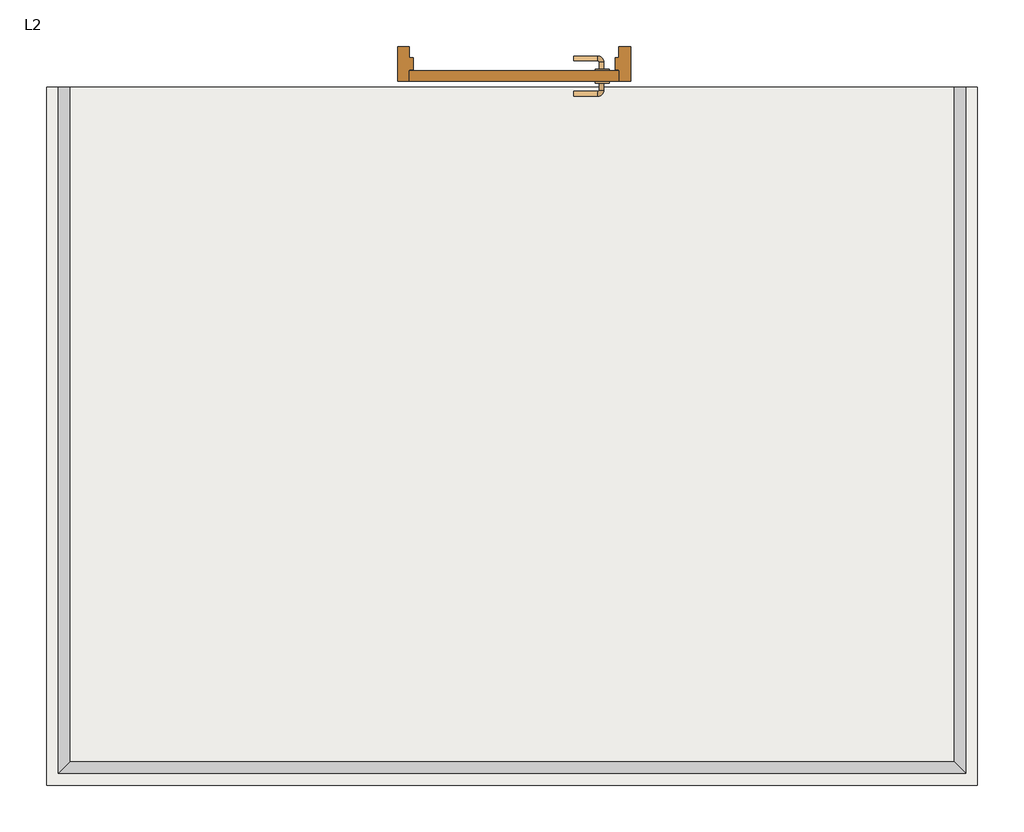
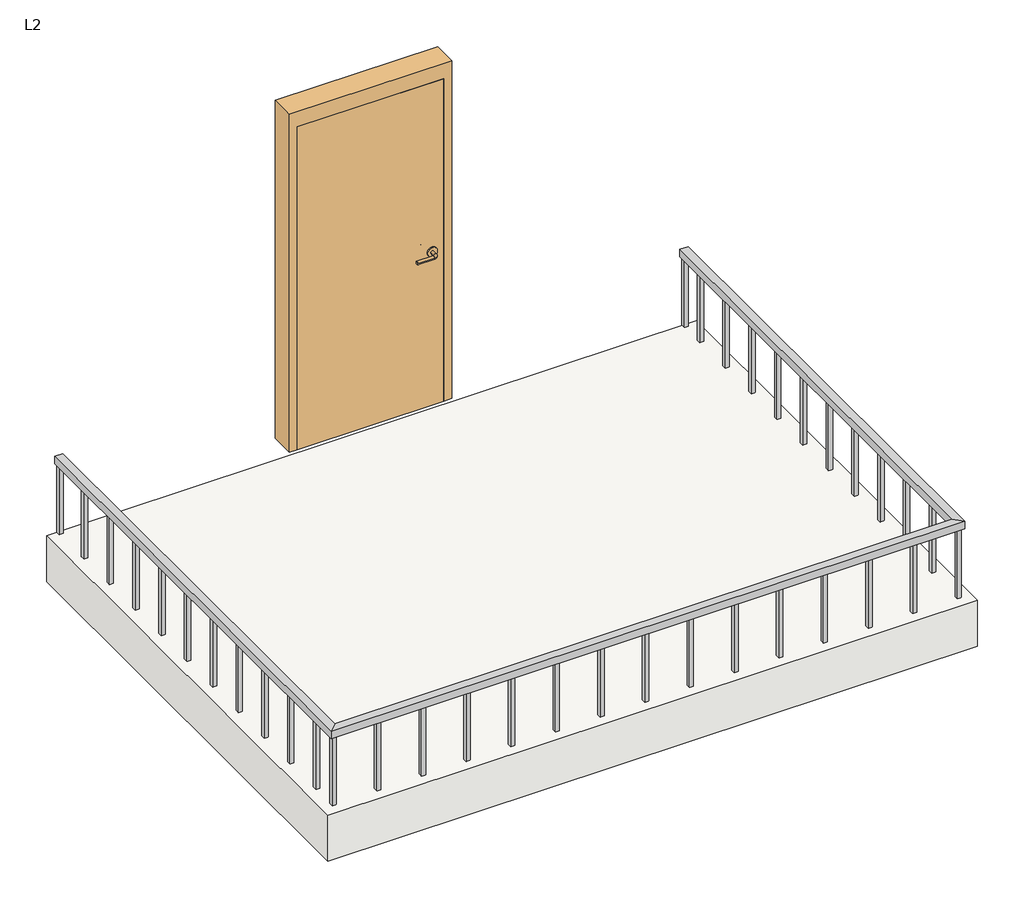
# One storey: 1 door, 1 railing, 1 slab.
"""IFC4 building model written with IfcOpenShell, lengths in millimetres."""

import ifcopenshell
import ifcopenshell.guid

model = None  # the IFC model being written
_history = None  # IfcOwnerHistory: only IFC2X3 demands one
_inside = {}  # id of a spatial element -> (the spatial element, [elements in it])
_under = {}  # id of a project, library or spatial element -> (it, [spatial elements below it])
_declared = {}  # id of a project -> (the project, [libraries it declares])
_typed = {}  # id of a type object -> (the type object, [elements of that type])
_made_of = {}  # id of a material, layer set ... -> (it, [elements and type objects made of it])


def new_model(schema):
    """Start an empty IFC model of exactly this schema.

    Asked for "IFC4X3", IfcOpenShell would pick the latest addendum, in which some entities
    have other attributes; the version numbers below select the first issue.
    IFC2X3 requires an IfcOwnerHistory on every rooted entity: one is made here for all.
    """
    global model, _history
    if schema == "IFC4X3":
        model = ifcopenshell.file(schema_version=(4, 3, 0, 0))
    else:
        model = ifcopenshell.file(schema=schema)
    _inside.clear()
    _under.clear()
    _declared.clear()
    _typed.clear()
    _made_of.clear()
    _history = None
    if model.schema == "IFC2X3":
        org = make("IfcOrganization", Name="unknown")
        user = make(
            "IfcPersonAndOrganization",
            ThePerson=make("IfcPerson", FamilyName="unknown"),
            TheOrganization=org,
        )
        app = make(
            "IfcApplication",
            ApplicationDeveloper=org,
            Version="unknown",
            ApplicationFullName="unknown",
            ApplicationIdentifier="unknown",
        )
        _history = make(
            "IfcOwnerHistory",
            OwningUser=user,
            OwningApplication=app,
            ChangeAction="ADDED",
            CreationDate=0,
        )
    return model


def make(cls, **values):
    """One entity of the class cls with the attributes given. An attribute that is None is left unset."""
    return model.create_entity(
        cls, **{name: value for name, value in values.items() if value is not None}
    )


def rooted(cls, **values):
    """An entity with a GlobalId (a new one), such as an element, a storey or a relation."""
    return make(cls, GlobalId=ifcopenshell.guid.new(), OwnerHistory=_history, **values)


def si_unit(unit_type, name, prefix=None):
    """IfcSIUnit, for example si_unit("LENGTHUNIT", "METRE", prefix="MILLI")."""
    return make("IfcSIUnit", UnitType=unit_type, Prefix=prefix, Name=name)


def assignment(units):
    """IfcUnitAssignment: the units of a project."""
    return None if units is None else make("IfcUnitAssignment", Units=units)


def point(xyz):
    """IfcCartesianPoint."""
    return None if xyz is None else make("IfcCartesianPoint", Coordinates=xyz)


def direction(xyz):
    """IfcDirection."""
    return None if xyz is None else make("IfcDirection", DirectionRatios=xyz)


def frame(location, z_axis=None, x_axis=None):
    """IfcAxis2Placement3D, a coordinate frame: its origin and axes. An axis left out is left unset."""
    return make(
        "IfcAxis2Placement3D",
        Location=point(location),
        Axis=direction(z_axis),
        RefDirection=direction(x_axis),
    )


def frame_2d(location, x_axis=None):
    """IfcAxis2Placement2D, a coordinate frame in the plane: its origin and x axis."""
    return make(
        "IfcAxis2Placement2D", Location=point(location), RefDirection=direction(x_axis)
    )


def origin():
    """The frame at (0, 0, 0) with its axes left unset."""
    return frame((0.0, 0.0, 0.0))


def origin_with_axes():
    """The frame at (0, 0, 0) with the z axis (0, 0, 1) and the x axis (1, 0, 0) written out."""
    return frame((0.0, 0.0, 0.0), z_axis=(0.0, 0.0, 1.0), x_axis=(1.0, 0.0, 0.0))


def place(relative_to, where):
    """IfcLocalPlacement: puts the frame where relative to a parent placement (None: the world)."""
    return make(
        "IfcLocalPlacement", PlacementRelTo=relative_to, RelativePlacement=where
    )


def context(
    kind, dimensions, precision=None, world=None, true_north=None, identifier=None
):
    """IfcGeometricRepresentationContext, for example the 3D "Model" context."""
    return make(
        "IfcGeometricRepresentationContext",
        ContextIdentifier=identifier,
        ContextType=kind,
        CoordinateSpaceDimension=dimensions,
        Precision=precision,
        WorldCoordinateSystem=world,
        TrueNorth=true_north,
    )


def project(units=None, contexts=None):
    """IfcProject with its units and contexts."""
    return rooted(
        "IfcProject",
        Name="project",
        RepresentationContexts=contexts,
        UnitsInContext=assignment(units),
    )


def spatial(cls, under=None, at=None, **own):
    """A site, building, storey or space (cls), placed at a placement, below another one or the project."""
    s = rooted(cls, ObjectPlacement=at, **own)
    if under is not None:
        _under.setdefault(under.id(), (under, []))[1].append(s)
    return s


def polyline(points):
    """IfcPolyline through the points."""
    return make("IfcPolyline", Points=[point(p) for p in points])


def circle_curve(where, radius):
    """IfcCircle in the frame where."""
    return make("IfcCircle", Position=where, Radius=radius)


def ellipse_curve(where, semi_axis1, semi_axis2):
    """IfcEllipse in the frame where."""
    return make(
        "IfcEllipse", Position=where, SemiAxis1=semi_axis1, SemiAxis2=semi_axis2
    )


def trimmed(basis, trim1, trim2, sense, master):
    """IfcTrimmedCurve: the piece of a basis curve between two trims."""
    return make(
        "IfcTrimmedCurve",
        BasisCurve=basis,
        Trim1=trim1,
        Trim2=trim2,
        SenseAgreement=sense,
        MasterRepresentation=master,
    )


def segment(curve, same_sense, transition):
    """IfcCompositeCurveSegment."""
    return make(
        "IfcCompositeCurveSegment",
        Transition=transition,
        SameSense=same_sense,
        ParentCurve=curve,
    )


def composite_curve(segments, self_intersect=None):
    """IfcCompositeCurve: segments joined end to end."""
    return make("IfcCompositeCurve", Segments=segments, SelfIntersect=self_intersect)


def outline(outer, holes=None, kind="AREA"):
    """IfcArbitraryClosedProfileDef: a profile drawn as a closed curve; with holes, ...WithVoids."""
    if holes is None:
        return make("IfcArbitraryClosedProfileDef", ProfileType=kind, OuterCurve=outer)
    return make(
        "IfcArbitraryProfileDefWithVoids",
        ProfileType=kind,
        OuterCurve=outer,
        InnerCurves=holes,
    )


def extrude(swept, where, along, depth):
    """IfcExtrudedAreaSolid: the profile swept, set in the frame where, extruded along a direction by depth."""
    return make(
        "IfcExtrudedAreaSolid",
        SweptArea=swept,
        Position=where,
        ExtrudedDirection=direction(along),
        Depth=depth,
    )


def faces_of(points, faces, orient=None, outer=None):
    """IfcFace entities. A face is a list of loops; a loop is a list of indices into points, from 0.

    orient and outer hold one flag for each loop. By default every Orientation is true, the
    first loop of a face is its IfcFaceOuterBound and the others are IfcFaceBound.
    """
    made = []
    for i, loops in enumerate(faces):
        bounds = []
        for j, loop in enumerate(loops):
            is_outer = j == 0 if outer is None else outer[i][j]
            bounds.append(
                make(
                    "IfcFaceOuterBound" if is_outer else "IfcFaceBound",
                    Bound=make("IfcPolyLoop", Polygon=[points[k] for k in loop]),
                    Orientation=True if orient is None else orient[i][j],
                )
            )
        made.append(make("IfcFace", Bounds=bounds))
    return made


def faceted_brep(points, faces, orient=None, outer=None, voids=None):
    """IfcFacetedBrep: a solid bounded by flat faces; with voids (closed shells), ...WithVoids."""
    shared = [point(p) for p in points]
    hull = make("IfcClosedShell", CfsFaces=faces_of(shared, faces, orient, outer))
    if voids is None:
        return make("IfcFacetedBrep", Outer=hull)
    return make(
        "IfcFacetedBrepWithVoids",
        Outer=hull,
        Voids=[
            make(cls, CfsFaces=faces_of(shared, fs, o, b)) for cls, fs, o, b in voids
        ],
    )


def shape(context_of_items, identifier, shape_type, items):
    """IfcShapeRepresentation: the items that make up one representation, for example the "Body"."""
    return make(
        "IfcShapeRepresentation",
        ContextOfItems=context_of_items,
        RepresentationIdentifier=identifier,
        RepresentationType=shape_type,
        Items=items,
    )


def source(mapping_origin, context_of_items, identifier, shape_type, items):
    """IfcRepresentationMap: a shape defined once, which mapped items show again and again."""
    return make(
        "IfcRepresentationMap",
        MappingOrigin=mapping_origin,
        MappedRepresentation=shape(context_of_items, identifier, shape_type, items),
    )


def transform(
    local_origin,
    x_axis=None,
    y_axis=None,
    z_axis=None,
    scale=None,
    scale2=None,
    scale3=None,
    uniform=True,
):
    """IfcCartesianTransformationOperator3D, or its non-uniform kind. x_axis, y_axis, z_axis: its Axis1, 2, 3."""
    if uniform:
        return make(
            "IfcCartesianTransformationOperator3D",
            Axis1=direction(x_axis),
            Axis2=direction(y_axis),
            LocalOrigin=point(local_origin),
            Scale=scale,
            Axis3=direction(z_axis),
        )
    return make(
        "IfcCartesianTransformationOperator3DnonUniform",
        Axis1=direction(x_axis),
        Axis2=direction(y_axis),
        LocalOrigin=point(local_origin),
        Scale=scale,
        Axis3=direction(z_axis),
        Scale2=scale2,
        Scale3=scale3,
    )


def mapped(mapping_source, mapping_target):
    """IfcMappedItem: shows the shape of a source again, moved by a transform."""
    return make(
        "IfcMappedItem", MappingSource=mapping_source, MappingTarget=mapping_target
    )


def made_of(thing, what):
    """Note that an element or type object is made of a material, layer set ...; save() writes the relation."""
    if what is not None:
        _made_of.setdefault(what.id(), (what, []))[1].append(thing)
    return thing


def element(
    cls,
    number,
    at=None,
    inside=None,
    cuts=None,
    type_object=None,
    material=None,
    context=None,
    identifier="Body",
    shape_type=None,
    held_by="IfcProductDefinitionShape",
    body=None,
    shapes=None,
    **own,
):
    """One element of the class cls, such as IfcWall. Its Tag is "e" and its number.

    at: its placement. inside: the storey or other place that contains it. cuts: it is an
    opening in that element (IfcRelVoidsElement). A single representation is given by context,
    identifier, shape_type and body (its items); several are given by shapes. held_by: the class
    of the entity that holds the representations. save() writes the other relations.
    """
    e = rooted(cls, Tag="e%d" % number, ObjectPlacement=at, **own)
    if body is not None:
        shapes = [shape(context, identifier, shape_type, body)]
    if shapes is not None:
        e.Representation = make(held_by, Representations=shapes)
    if inside is not None:
        _inside.setdefault(inside.id(), (inside, []))[1].append(e)
    if cuts is not None:
        rooted(
            "IfcRelVoidsElement", RelatingBuildingElement=cuts, RelatedOpeningElement=e
        )
    if type_object is not None:
        _typed.setdefault(type_object.id(), (type_object, []))[1].append(e)
    return made_of(e, material)


def aggregate(whole, parts):
    """IfcRelAggregates: a whole, such as a stair, and the parts it consists of."""
    return rooted("IfcRelAggregates", RelatingObject=whole, RelatedObjects=parts)


def save(model, path):
    """Write the relations noted so far, then the file.

    IfcRelAggregates (storeys below a building ...), IfcRelContainedInSpatialStructure (elements
    in a storey), IfcRelDefinesByType, IfcRelAssociatesMaterial and IfcRelDeclares: one each for
    every whole, place, type object, material and project.
    """
    for whole, parts in _under.values():
        aggregate(whole, parts)
    for where, things in _inside.values():
        rooted(
            "IfcRelContainedInSpatialStructure",
            RelatedElements=things,
            RelatingStructure=where,
        )
    for kind, things in _typed.values():
        rooted("IfcRelDefinesByType", RelatedObjects=things, RelatingType=kind)
    for what, things in _made_of.values():
        rooted("IfcRelAssociatesMaterial", RelatedObjects=things, RelatingMaterial=what)
    for by, libraries in _declared.values():
        rooted("IfcRelDeclares", RelatingContext=by, RelatedDefinitions=libraries)
    model.write(path)


def plane_surface(at):
    """IfcPlane: the flat surface through the origin of the frame at, square to its z axis."""
    return make("IfcPlane", Position=at)


def cylinder_surface(at, radius):
    """IfcCylindricalSurface: all points at the distance radius from the z axis of the frame at."""
    return make("IfcCylindricalSurface", Position=at, Radius=radius)


def revolved_surface(curve, axis_point, axis_direction):
    """IfcSurfaceOfRevolution: the curve turned about the line through axis_point along axis_direction."""
    return make(
        "IfcSurfaceOfRevolution",
        SweptCurve=make("IfcArbitraryOpenProfileDef", ProfileType="CURVE", Curve=curve),
        AxisPosition=make("IfcAxis1Placement", Location=point(axis_point), Axis=direction(axis_direction)),
    )


def advanced_brep(points, edges, surfaces, faces):
    """IfcAdvancedBrep: a solid bounded by faces that lie on surfaces and meet in shared edges.

    An edge is (start, end): straight between two places in points (the first is 0);
    or (start, end, curve); or (start, end, curve, False) where it runs against its curve.
    A face is (place in surfaces, loops), or (place, loops, False) where it looks against
    its surface's normal. A loop lists edges by number (the first is 1), with a minus sign
    where the edge is run from its end to its start. The first loop is the outer one.
    """
    corners = [point(p) for p in points]
    vertices = [make("IfcVertexPoint", VertexGeometry=c) for c in corners]
    made = []
    for start, end, *more in edges:
        made.append(
            make(
                "IfcEdgeCurve",
                EdgeStart=vertices[start],
                EdgeEnd=vertices[end],
                EdgeGeometry=more[0] if more else make("IfcPolyline", Points=[corners[start], corners[end]]),
                SameSense=more[1] if len(more) > 1 else True,
            )
        )
    hull = []
    for where, loops, *sense in faces:
        bounds = []
        for j, loop in enumerate(loops):
            ring = [make("IfcOrientedEdge", EdgeElement=made[abs(k) - 1], Orientation=k > 0) for k in loop]
            bounds.append(
                make(
                    "IfcFaceOuterBound" if j == 0 else "IfcFaceBound",
                    Bound=make("IfcEdgeLoop", EdgeList=ring),
                    Orientation=True,
                )
            )
        hull.append(make("IfcAdvancedFace", Bounds=bounds, FaceSurface=surfaces[where], SameSense=sense[0] if sense else True))
    return make("IfcAdvancedBrep", Outer=make("IfcClosedShell", CfsFaces=hull))


def m_door_passage_single_flush_900_x_2100mm_f70d95c9(model_context):
    return source(origin(), model_context, "Body", "SolidModel", [
        advanced_brep(
        [(-384.990625, 3.35, 1000.0), (-364.990625, 3.35, 1000.0), (-364.990625, -26.65, 1000.0), (-384.990625, -26.65, 1000.0), (-359.990625, -31.65, 1000.0), (-359.990625, -51.65, 1000.0), (-254.990625, -51.65, 1000.0), (-254.990625, -31.65, 1000.0)],
        [
            (0, 1, circle_curve(frame((-374.990625, 3.35, 1000.0), z_axis=(0.0, 1.0, 0.0), x_axis=(1.0, 0.0, 0.0)), 10.0)),
            (1, 0, circle_curve(frame((-374.990625, 3.35, 1000.0), z_axis=(0.0, 1.0, 0.0), x_axis=(1.0, 0.0, 0.0)), 10.0)),
            (1, 2),
            (2, 3, circle_curve(frame((-374.990625, -26.65, 1000.0), z_axis=(0.0, 1.0, 0.0), x_axis=(1.0, 0.0, 0.0)), 10.0)),
            (3, 0),
            (3, 2, circle_curve(frame((-374.990625, -26.65, 1000.0), z_axis=(0.0, 1.0, 0.0), x_axis=(1.0, 0.0, 0.0)), 10.0)),
            (4, 5, circle_curve(frame((-359.990625, -41.65, 1000.0), z_axis=(-1.0, 0.0, 0.0), x_axis=(0.0, 1.0, 0.0)), 10.0)),
            (5, 3, circle_curve(frame((-359.990625, -26.65, 1000.0), z_axis=(0.0, 0.0, -1.0), x_axis=(-1.0, 0.0, 0.0)), 25.0)),
            (2, 4, circle_curve(frame((-359.990625, -26.65, 1000.0), z_axis=(0.0, 0.0, 1.0), x_axis=(-1.0, 0.0, 0.0)), 5.0)),
            (5, 4, circle_curve(frame((-359.990625, -41.65, 1000.0), z_axis=(-1.0, 0.0, 0.0), x_axis=(0.0, 1.0, 0.0)), 10.0)),
            (6, 7, circle_curve(frame((-254.990625, -41.65, 1000.0), z_axis=(1.0, 0.0, 0.0), x_axis=(0.0, 1.0, 0.0)), 10.0)),
            (7, 6, circle_curve(frame((-254.990625, -41.65, 1000.0), z_axis=(1.0, 0.0, 0.0), x_axis=(0.0, 1.0, 0.0)), 10.0)),
            (4, 7),
            (6, 5),
        ],
        [
            plane_surface(frame((-374.990625, 3.35, 1000.0), z_axis=(0.0, 1.0, 0.0), x_axis=(0.0, 0.0, 1.0))),
            cylinder_surface(frame((-374.990625, 3.35, 1000.0), z_axis=(0.0, 1.0, 0.0), x_axis=(1.0, 0.0, 0.0)), 10.0),
            revolved_surface(trimmed(ellipse_curve(frame((-374.990625, -26.65, 1000.0), z_axis=(0.0, -1.0, 0.0), x_axis=(1.0, 0.0, 0.0)), 10.0, 10.0), [point((-384.990625, -26.65, 1000.0))], [point((-364.990625, -26.65, 1000.0))], True, "CARTESIAN"), (-359.990625, -26.65, 1000.0), (0.0, 0.0, -1.0)),
            revolved_surface(trimmed(ellipse_curve(frame((-374.990625, -26.65, 1000.0), z_axis=(0.0, -1.0, 0.0), x_axis=(1.0, 0.0, 0.0)), 10.0, 10.0), [point((-364.990625, -26.65, 1000.0))], [point((-384.990625, -26.65, 1000.0))], True, "CARTESIAN"), (-359.990625, -26.65, 1000.0), (0.0, 0.0, -1.0)),
            plane_surface(frame((-254.990625, -41.65, 1000.0), z_axis=(1.0, 0.0, 0.0), x_axis=(0.0, 0.0, 1.0))),
            cylinder_surface(frame((-359.990625, -41.65, 1000.0), z_axis=(-1.0, 0.0, 0.0), x_axis=(0.0, 1.0, 0.0)), 10.0),
        ],
        [
            (0, [[1, 2]]),
            (1, [[3, 4, 5, -2]]),
            (1, [[-5, 6, -3, -1]]),
            (2, [[7, 8, -4, 9]]),
            (3, [[10, -9, -6, -8]]),
            (4, [[11, 12]]),
            (5, [[13, -11, 14, -7]]),
            (5, [[-14, -12, -13, -10]]),
        ],
    ),
        extrude(outline(composite_curve([segment(trimmed(circle_curve(frame_2d((1000.0, -377.490625)), 30.0), [point((1000.0, -407.490625))], [point((1000.0, -347.490625))], False, "CARTESIAN"), True, "CONTINUOUS"), segment(trimmed(circle_curve(frame_2d((1000.0, -377.490625)), 30.0), [point((1000.0, -347.490625))], [point((1000.0, -407.490625))], False, "CARTESIAN"), True, "CONTINUOUS")], self_intersect=False)), frame((0.0, 3.35, 0.0), z_axis=(0.0, 1.0, 0.0), x_axis=(0.0, 0.0, 1.0)), (0.0, 0.0, 1.0), 8.0),
        advanced_brep(
        [(-384.990625, 64.35, 1000.0), (-364.990625, 64.35, 1000.0), (-384.990625, 94.35, 1000.0), (-364.990625, 94.35, 1000.0), (-359.990625, 99.35, 1000.0), (-359.990625, 119.35, 1000.0), (-254.990625, 119.35, 1000.0), (-254.990625, 99.35, 1000.0)],
        [
            (0, 1, circle_curve(frame((-374.990625, 64.35, 1000.0), z_axis=(0.0, -1.0, 0.0), x_axis=(1.0, 0.0, 0.0)), 10.0)),
            (1, 0, circle_curve(frame((-374.990625, 64.35, 1000.0), z_axis=(0.0, -1.0, 0.0), x_axis=(1.0, 0.0, 0.0)), 10.0)),
            (0, 2),
            (2, 3, circle_curve(frame((-374.990625, 94.35, 1000.0), z_axis=(0.0, -1.0, 0.0), x_axis=(1.0, 0.0, 0.0)), 10.0)),
            (3, 1),
            (3, 2, circle_curve(frame((-374.990625, 94.35, 1000.0), z_axis=(0.0, -1.0, 0.0), x_axis=(1.0, 0.0, 0.0)), 10.0)),
            (4, 3, circle_curve(frame((-359.990625, 94.35, 1000.0), z_axis=(0.0, 0.0, 1.0), x_axis=(-1.0, 0.0, 0.0)), 5.0)),
            (2, 5, circle_curve(frame((-359.990625, 94.35, 1000.0), z_axis=(0.0, 0.0, -1.0), x_axis=(-1.0, 0.0, 0.0)), 25.0)),
            (5, 4, circle_curve(frame((-359.990625, 109.35, 1000.0), z_axis=(-1.0, 0.0, 0.0), x_axis=(0.0, -1.0, 0.0)), 10.0)),
            (4, 5, circle_curve(frame((-359.990625, 109.35, 1000.0), z_axis=(-1.0, 0.0, 0.0), x_axis=(0.0, -1.0, 0.0)), 10.0)),
            (6, 7, circle_curve(frame((-254.990625, 109.35, 1000.0), z_axis=(1.0, 0.0, 0.0), x_axis=(0.0, -1.0, 0.0)), 10.0)),
            (7, 6, circle_curve(frame((-254.990625, 109.35, 1000.0), z_axis=(1.0, 0.0, 0.0), x_axis=(0.0, -1.0, 0.0)), 10.0)),
            (5, 6),
            (7, 4),
        ],
        [
            plane_surface(frame((-374.990625, 64.35, 1000.0), z_axis=(0.0, -1.0, 0.0), x_axis=(0.0, 0.0, 1.0))),
            cylinder_surface(frame((-374.990625, 64.35, 1000.0), z_axis=(0.0, -1.0, 0.0), x_axis=(1.0, 0.0, 0.0)), 10.0),
            revolved_surface(trimmed(ellipse_curve(frame((-374.990625, 94.35, 1000.0), z_axis=(0.0, -1.0, 0.0), x_axis=(1.0, 0.0, 0.0)), 10.0, 10.0), [point((-384.990625, 94.35, 1000.0))], [point((-364.990625, 94.35, 1000.0))], True, "CARTESIAN"), (-359.990625, 94.35, 1000.0), (0.0, 0.0, -1.0)),
            revolved_surface(trimmed(ellipse_curve(frame((-374.990625, 94.35, 1000.0), z_axis=(0.0, -1.0, 0.0), x_axis=(1.0, 0.0, 0.0)), 10.0, 10.0), [point((-364.990625, 94.35, 1000.0))], [point((-384.990625, 94.35, 1000.0))], True, "CARTESIAN"), (-359.990625, 94.35, 1000.0), (0.0, 0.0, -1.0)),
            plane_surface(frame((-254.990625, 109.35, 1000.0), z_axis=(1.0, 0.0, 0.0), x_axis=(0.0, 0.0, 1.0))),
            cylinder_surface(frame((-359.990625, 109.35, 1000.0), z_axis=(-1.0, 0.0, 0.0), x_axis=(0.0, -1.0, 0.0)), 10.0),
        ],
        [
            (0, [[1, 2]]),
            (1, [[-1, 3, 4, 5]]),
            (1, [[-2, -5, 6, -3]]),
            (2, [[7, -4, 8, 9]]),
            (3, [[-8, -6, -7, 10]]),
            (4, [[11, 12]]),
            (5, [[-9, 13, -12, 14]]),
            (5, [[-10, -14, -11, -13]]),
        ],
    ),
        extrude(outline(composite_curve([segment(trimmed(circle_curve(frame_2d((1000.0, -377.490625)), 30.0), [point((1000.0, -407.490625))], [point((1000.0, -347.490625))], False, "CARTESIAN"), True, "CONTINUOUS"), segment(trimmed(circle_curve(frame_2d((1000.0, -377.490625)), 30.0), [point((1000.0, -347.490625))], [point((1000.0, -407.490625))], False, "CARTESIAN"), True, "CONTINUOUS")], self_intersect=False)), frame((0.0, 56.35, 0.0), z_axis=(0.0, 1.0, 0.0), x_axis=(0.0, 0.0, 1.0)), (0.0, 0.0, 1.0), 8.0),
        extrude(outline(polyline([(450.0, 11.35), (-450.0, 11.35), (-450.0, 56.35), (450.0, 56.35), (450.0, 11.35)])), origin_with_axes(), (0.0, 0.0, 1.0), 2100.0),
        faceted_brep([(450.0, 6.5875, 0.0), (450.0, 56.35, 0.0), (500.0, 56.35, 0.0), (500.0, -93.65, 0.0), (450.0, -93.65, 0.0), (450.0, -44.4375, 0.0), (434.125, -44.4375, 0.0), (434.125, 6.5875, 0.0), (450.0, 6.5875, 2100.0), (450.0, 56.35, 2100.0), (-450.0, 56.35, 2100.0), (-450.0, 56.35, 0.0), (-500.0, 56.35, 0.0), (-500.0, 56.35, 2200.0), (500.0, 56.35, 2200.0), (500.0, -93.65, 2200.0), (-500.0, -93.65, 2200.0), (-500.0, -93.65, 0.0), (-450.0, -93.65, 0.0), (-450.0, -93.65, 2100.0), (450.0, -93.65, 2100.0), (450.0, -44.4375, 2100.0), (-450.0, -44.4375, 2100.0), (-450.0, -44.4375, 0.0), (-434.125, -44.4375, 0.0), (-434.125, -44.4375, 2084.125), (434.125, -44.4375, 2084.125), (434.125, 6.5875, 2084.125), (-434.125, 6.5875, 2084.125), (-434.125, 6.5875, 0.0), (-450.0, 6.5875, 0.0), (-450.0, 6.5875, 2100.0)], [[[0, 1, 2, 3, 4, 5, 6, 7]], [[1, 0, 8, 9]], [[2, 1, 9, 10, 11, 12, 13, 14]], [[3, 2, 14, 15]], [[4, 3, 15, 16, 17, 18, 19, 20]], [[5, 4, 20, 21]], [[6, 5, 21, 22, 23, 24, 25, 26]], [[7, 6, 26, 27]], [[0, 7, 27, 28, 29, 30, 31, 8]], [[9, 8, 31, 10]], [[20, 19, 22, 21]], [[26, 25, 28, 27]], [[12, 11, 30, 29, 24, 23, 18, 17]], [[11, 10, 31, 30]], [[13, 12, 17, 16]], [[19, 18, 23, 22]], [[25, 24, 29, 28]], [[15, 14, 13, 16]]]),
    ])


model = new_model("IFC4")

# Units and contexts
model_context = context("Model", 3, world=origin())
ifc_project = project(units=[si_unit("LENGTHUNIT", "METRE", prefix="MILLI")], contexts=[model_context])

# Site, building, storey
site = spatial("IfcSite", under=ifc_project)
building = spatial("IfcBuilding", under=site)
storey = spatial("IfcBuildingStorey", under=building, Name="L2", Elevation=1200.0)

# Door
placement = place(None, origin())
m_door_passage_single_flush_900_x_2100mm_shape = m_door_passage_single_flush_900_x_2100mm_f70d95c9(model_context)
element("IfcDoor", 1, ObjectType="M_Door-Passage-Single-Flush : 900 x 2100mm", at=placement, inside=storey, context=model_context, shape_type="MappedRepresentation", body=[
    mapped(m_door_passage_single_flush_900_x_2100mm_shape, transform((752.7568, 2222.9207088, 1200.0), x_axis=(-1.0, 0.0, 0.0), y_axis=(0.0, -1.0, 0.0), z_axis=(0.0, 0.0, 1.0))),
])

# Railing
element("IfcRailing", 2, ObjectType="1100mm", at=placement, inside=storey, context=model_context, shape_type="SolidModel", body=[
    faceted_brep([(-1156.7682, 2141.5707088, 1700.0), (-1156.7682, 2141.5707088, 1650.0), (-1206.7682, 2141.5707088, 1650.0), (-1206.7682, 2141.5707088, 1700.0), (-1156.7682, -758.4292912, 1700.0), (-1156.7682, -758.4292912, 1650.0), (-1206.7682, -808.4292912, 1650.0), (-1206.7682, -808.4292912, 1700.0), (2643.2318, -758.4292912, 1700.0), (2643.2318, -758.4292912, 1650.0), (2693.2318, -808.4292912, 1650.0), (2693.2318, -808.4292912, 1700.0), (2643.2318, 2141.5707088, 1700.0), (2693.2318, 2141.5707088, 1700.0), (2693.2318, 2141.5707088, 1650.0), (2643.2318, 2141.5707088, 1650.0)], [[[0, 1, 2, 3]], [[1, 0, 4, 5]], [[2, 1, 5, 6]], [[3, 2, 6, 7]], [[0, 3, 7, 4]], [[5, 4, 8, 9]], [[6, 5, 9, 10]], [[7, 6, 10, 11]], [[4, 7, 11, 8]], [[12, 13, 14, 15]], [[9, 8, 12, 15]], [[10, 9, 15, 14]], [[11, 10, 14, 13]], [[8, 11, 13, 12]]]),
    extrude(outline(polyline([(2680.7318, 1954.0707088), (2655.7318, 1954.0707088), (2655.7318, 1979.0707088), (2680.7318, 1979.0707088), (2680.7318, 1954.0707088)])), frame((0.0, 0.0, 1200.0), z_axis=(0.0, 0.0, 1.0), x_axis=(1.0, 0.0, 0.0)), (0.0, 0.0, 1.0), 450.0),
    extrude(outline(polyline([(2680.7318, 1679.0707088), (2655.7318, 1679.0707088), (2655.7318, 1704.0707088), (2680.7318, 1704.0707088), (2680.7318, 1679.0707088)])), frame((0.0, 0.0, 1200.0), z_axis=(0.0, 0.0, 1.0), x_axis=(1.0, 0.0, 0.0)), (0.0, 0.0, 1.0), 450.0),
    extrude(outline(polyline([(2680.7318, 1404.0707088), (2655.7318, 1404.0707088), (2655.7318, 1429.0707088), (2680.7318, 1429.0707088), (2680.7318, 1404.0707088)])), frame((0.0, 0.0, 1200.0), z_axis=(0.0, 0.0, 1.0), x_axis=(1.0, 0.0, 0.0)), (0.0, 0.0, 1.0), 450.0),
    extrude(outline(polyline([(2680.7318, 1129.0707088), (2655.7318, 1129.0707088), (2655.7318, 1154.0707088), (2680.7318, 1154.0707088), (2680.7318, 1129.0707088)])), frame((0.0, 0.0, 1200.0), z_axis=(0.0, 0.0, 1.0), x_axis=(1.0, 0.0, 0.0)), (0.0, 0.0, 1.0), 450.0),
    extrude(outline(polyline([(2680.7318, 854.0707088), (2655.7318, 854.0707088), (2655.7318, 879.0707088), (2680.7318, 879.0707088), (2680.7318, 854.0707088)])), frame((0.0, 0.0, 1200.0), z_axis=(0.0, 0.0, 1.0), x_axis=(1.0, 0.0, 0.0)), (0.0, 0.0, 1.0), 450.0),
    extrude(outline(polyline([(2680.7318, 579.0707088), (2655.7318, 579.0707088), (2655.7318, 604.0707088), (2680.7318, 604.0707088), (2680.7318, 579.0707088)])), frame((0.0, 0.0, 1200.0), z_axis=(0.0, 0.0, 1.0), x_axis=(1.0, 0.0, 0.0)), (0.0, 0.0, 1.0), 450.0),
    extrude(outline(polyline([(2680.7318, 304.0707088), (2655.7318, 304.0707088), (2655.7318, 329.0707088), (2680.7318, 329.0707088), (2680.7318, 304.0707088)])), frame((0.0, 0.0, 1200.0), z_axis=(0.0, 0.0, 1.0), x_axis=(1.0, 0.0, 0.0)), (0.0, 0.0, 1.0), 450.0),
    extrude(outline(polyline([(2680.7318, 29.0707088), (2655.7318, 29.0707088), (2655.7318, 54.0707088), (2680.7318, 54.0707088), (2680.7318, 29.0707088)])), frame((0.0, 0.0, 1200.0), z_axis=(0.0, 0.0, 1.0), x_axis=(1.0, 0.0, 0.0)), (0.0, 0.0, 1.0), 450.0),
    extrude(outline(polyline([(2680.7318, -245.9292912), (2655.7318, -245.9292912), (2655.7318, -220.9292912), (2680.7318, -220.9292912), (2680.7318, -245.9292912)])), frame((0.0, 0.0, 1200.0), z_axis=(0.0, 0.0, 1.0), x_axis=(1.0, 0.0, 0.0)), (0.0, 0.0, 1.0), 450.0),
    extrude(outline(polyline([(2680.7318, -520.9292912), (2655.7318, -520.9292912), (2655.7318, -495.9292912), (2680.7318, -495.9292912), (2680.7318, -520.9292912)])), frame((0.0, 0.0, 1200.0), z_axis=(0.0, 0.0, 1.0), x_axis=(1.0, 0.0, 0.0)), (0.0, 0.0, 1.0), 450.0),
    extrude(outline(polyline([(2380.7318, -795.9292912), (2380.7318, -770.9292912), (2405.7318, -770.9292912), (2405.7318, -795.9292912), (2380.7318, -795.9292912)])), frame((0.0, 0.0, 1200.0), z_axis=(0.0, 0.0, 1.0), x_axis=(1.0, 0.0, 0.0)), (0.0, 0.0, 1.0), 450.0),
    extrude(outline(polyline([(2105.7318, -795.9292912), (2105.7318, -770.9292912), (2130.7318, -770.9292912), (2130.7318, -795.9292912), (2105.7318, -795.9292912)])), frame((0.0, 0.0, 1200.0), z_axis=(0.0, 0.0, 1.0), x_axis=(1.0, 0.0, 0.0)), (0.0, 0.0, 1.0), 450.0),
    extrude(outline(polyline([(1830.7318, -795.9292912), (1830.7318, -770.9292912), (1855.7318, -770.9292912), (1855.7318, -795.9292912), (1830.7318, -795.9292912)])), frame((0.0, 0.0, 1200.0), z_axis=(0.0, 0.0, 1.0), x_axis=(1.0, 0.0, 0.0)), (0.0, 0.0, 1.0), 450.0),
    extrude(outline(polyline([(1555.7318, -795.9292912), (1555.7318, -770.9292912), (1580.7318, -770.9292912), (1580.7318, -795.9292912), (1555.7318, -795.9292912)])), frame((0.0, 0.0, 1200.0), z_axis=(0.0, 0.0, 1.0), x_axis=(1.0, 0.0, 0.0)), (0.0, 0.0, 1.0), 450.0),
    extrude(outline(polyline([(1280.7318, -795.9292912), (1280.7318, -770.9292912), (1305.7318, -770.9292912), (1305.7318, -795.9292912), (1280.7318, -795.9292912)])), frame((0.0, 0.0, 1200.0), z_axis=(0.0, 0.0, 1.0), x_axis=(1.0, 0.0, 0.0)), (0.0, 0.0, 1.0), 450.0),
    extrude(outline(polyline([(1005.7318, -795.9292912), (1005.7318, -770.9292912), (1030.7318, -770.9292912), (1030.7318, -795.9292912), (1005.7318, -795.9292912)])), frame((0.0, 0.0, 1200.0), z_axis=(0.0, 0.0, 1.0), x_axis=(1.0, 0.0, 0.0)), (0.0, 0.0, 1.0), 450.0),
    extrude(outline(polyline([(730.7318, -795.9292912), (730.7318, -770.9292912), (755.7318, -770.9292912), (755.7318, -795.9292912), (730.7318, -795.9292912)])), frame((0.0, 0.0, 1200.0), z_axis=(0.0, 0.0, 1.0), x_axis=(1.0, 0.0, 0.0)), (0.0, 0.0, 1.0), 450.0),
    extrude(outline(polyline([(455.7318, -795.9292912), (455.7318, -770.9292912), (480.7318, -770.9292912), (480.7318, -795.9292912), (455.7318, -795.9292912)])), frame((0.0, 0.0, 1200.0), z_axis=(0.0, 0.0, 1.0), x_axis=(1.0, 0.0, 0.0)), (0.0, 0.0, 1.0), 450.0),
    extrude(outline(polyline([(180.7318, -795.9292912), (180.7318, -770.9292912), (205.7318, -770.9292912), (205.7318, -795.9292912), (180.7318, -795.9292912)])), frame((0.0, 0.0, 1200.0), z_axis=(0.0, 0.0, 1.0), x_axis=(1.0, 0.0, 0.0)), (0.0, 0.0, 1.0), 450.0),
    extrude(outline(polyline([(-94.2682, -795.9292912), (-94.2682, -770.9292912), (-69.2682, -770.9292912), (-69.2682, -795.9292912), (-94.2682, -795.9292912)])), frame((0.0, 0.0, 1200.0), z_axis=(0.0, 0.0, 1.0), x_axis=(1.0, 0.0, 0.0)), (0.0, 0.0, 1.0), 450.0),
    extrude(outline(polyline([(-369.2682, -795.9292912), (-369.2682, -770.9292912), (-344.2682, -770.9292912), (-344.2682, -795.9292912), (-369.2682, -795.9292912)])), frame((0.0, 0.0, 1200.0), z_axis=(0.0, 0.0, 1.0), x_axis=(1.0, 0.0, 0.0)), (0.0, 0.0, 1.0), 450.0),
    extrude(outline(polyline([(-644.2682, -795.9292912), (-644.2682, -770.9292912), (-619.2682, -770.9292912), (-619.2682, -795.9292912), (-644.2682, -795.9292912)])), frame((0.0, 0.0, 1200.0), z_axis=(0.0, 0.0, 1.0), x_axis=(1.0, 0.0, 0.0)), (0.0, 0.0, 1.0), 450.0),
    extrude(outline(polyline([(-919.2682, -795.9292912), (-919.2682, -770.9292912), (-894.2682, -770.9292912), (-894.2682, -795.9292912), (-919.2682, -795.9292912)])), frame((0.0, 0.0, 1200.0), z_axis=(0.0, 0.0, 1.0), x_axis=(1.0, 0.0, 0.0)), (0.0, 0.0, 1.0), 450.0),
    extrude(outline(polyline([(-1194.2682, -595.9292912), (-1169.2682, -595.9292912), (-1169.2682, -620.9292912), (-1194.2682, -620.9292912), (-1194.2682, -595.9292912)])), frame((0.0, 0.0, 1200.0), z_axis=(0.0, 0.0, 1.0), x_axis=(1.0, 0.0, 0.0)), (0.0, 0.0, 1.0), 450.0),
    extrude(outline(polyline([(-1194.2682, -320.9292912), (-1169.2682, -320.9292912), (-1169.2682, -345.9292912), (-1194.2682, -345.9292912), (-1194.2682, -320.9292912)])), frame((0.0, 0.0, 1200.0), z_axis=(0.0, 0.0, 1.0), x_axis=(1.0, 0.0, 0.0)), (0.0, 0.0, 1.0), 450.0),
    extrude(outline(polyline([(-1194.2682, -45.9292912), (-1169.2682, -45.9292912), (-1169.2682, -70.9292912), (-1194.2682, -70.9292912), (-1194.2682, -45.9292912)])), frame((0.0, 0.0, 1200.0), z_axis=(0.0, 0.0, 1.0), x_axis=(1.0, 0.0, 0.0)), (0.0, 0.0, 1.0), 450.0),
    extrude(outline(polyline([(-1194.2682, 229.0707088), (-1169.2682, 229.0707088), (-1169.2682, 204.0707088), (-1194.2682, 204.0707088), (-1194.2682, 229.0707088)])), frame((0.0, 0.0, 1200.0), z_axis=(0.0, 0.0, 1.0), x_axis=(1.0, 0.0, 0.0)), (0.0, 0.0, 1.0), 450.0),
    extrude(outline(polyline([(-1194.2682, 504.0707088), (-1169.2682, 504.0707088), (-1169.2682, 479.0707088), (-1194.2682, 479.0707088), (-1194.2682, 504.0707088)])), frame((0.0, 0.0, 1200.0), z_axis=(0.0, 0.0, 1.0), x_axis=(1.0, 0.0, 0.0)), (0.0, 0.0, 1.0), 450.0),
    extrude(outline(polyline([(-1194.2682, 779.0707088), (-1169.2682, 779.0707088), (-1169.2682, 754.0707088), (-1194.2682, 754.0707088), (-1194.2682, 779.0707088)])), frame((0.0, 0.0, 1200.0), z_axis=(0.0, 0.0, 1.0), x_axis=(1.0, 0.0, 0.0)), (0.0, 0.0, 1.0), 450.0),
    extrude(outline(polyline([(-1194.2682, 1054.0707088), (-1169.2682, 1054.0707088), (-1169.2682, 1029.0707088), (-1194.2682, 1029.0707088), (-1194.2682, 1054.0707088)])), frame((0.0, 0.0, 1200.0), z_axis=(0.0, 0.0, 1.0), x_axis=(1.0, 0.0, 0.0)), (0.0, 0.0, 1.0), 450.0),
    extrude(outline(polyline([(-1194.2682, 1329.0707088), (-1169.2682, 1329.0707088), (-1169.2682, 1304.0707088), (-1194.2682, 1304.0707088), (-1194.2682, 1329.0707088)])), frame((0.0, 0.0, 1200.0), z_axis=(0.0, 0.0, 1.0), x_axis=(1.0, 0.0, 0.0)), (0.0, 0.0, 1.0), 450.0),
    extrude(outline(polyline([(-1194.2682, 1604.0707088), (-1169.2682, 1604.0707088), (-1169.2682, 1579.0707088), (-1194.2682, 1579.0707088), (-1194.2682, 1604.0707088)])), frame((0.0, 0.0, 1200.0), z_axis=(0.0, 0.0, 1.0), x_axis=(1.0, 0.0, 0.0)), (0.0, 0.0, 1.0), 450.0),
    extrude(outline(polyline([(-1194.2682, 1879.0707088), (-1169.2682, 1879.0707088), (-1169.2682, 1854.0707088), (-1194.2682, 1854.0707088), (-1194.2682, 1879.0707088)])), frame((0.0, 0.0, 1200.0), z_axis=(0.0, 0.0, 1.0), x_axis=(1.0, 0.0, 0.0)), (0.0, 0.0, 1.0), 450.0),
    extrude(outline(polyline([(2655.7318, -795.9292912), (2655.7318, -770.9292912), (2680.7318, -770.9292912), (2680.7318, -795.9292912), (2655.7318, -795.9292912)])), frame((0.0, 0.0, 1200.0), z_axis=(0.0, 0.0, 1.0), x_axis=(1.0, 0.0, 0.0)), (0.0, 0.0, 1.0), 450.0),
    extrude(outline(polyline([(-1194.2682, -770.9292912), (-1169.2682, -770.9292912), (-1169.2682, -795.9292912), (-1194.2682, -795.9292912), (-1194.2682, -770.9292912)])), frame((0.0, 0.0, 1200.0), z_axis=(0.0, 0.0, 1.0), x_axis=(1.0, 0.0, 0.0)), (0.0, 0.0, 1.0), 450.0),
    extrude(outline(polyline([(2680.7318, 2116.5707088), (2655.7318, 2116.5707088), (2655.7318, 2141.5707088), (2680.7318, 2141.5707088), (2680.7318, 2116.5707088)])), frame((0.0, 0.0, 1200.0), z_axis=(0.0, 0.0, 1.0), x_axis=(1.0, 0.0, 0.0)), (0.0, 0.0, 1.0), 450.0),
    extrude(outline(polyline([(-1194.2682, 2141.5707088), (-1169.2682, 2141.5707088), (-1169.2682, 2116.5707088), (-1194.2682, 2116.5707088), (-1194.2682, 2141.5707088)])), frame((0.0, 0.0, 1200.0), z_axis=(0.0, 0.0, 1.0), x_axis=(1.0, 0.0, 0.0)), (0.0, 0.0, 1.0), 450.0),
])

# Slab
element("IfcSlab", 3, ObjectType="Generic 300mm", at=placement, inside=storey, context=model_context, shape_type="SweptSolid", body=[
    extrude(outline(polyline([(2743.2318, -858.4292912), (-1256.7682, -858.4292912), (-1256.7682, 2141.5707088), (2743.2318, 2141.5707088), (2743.2318, -858.4292912)])), frame((0.0, 0.0, 900.0), z_axis=(0.0, 0.0, 1.0), x_axis=(1.0, 0.0, 0.0)), (0.0, 0.0, 1.0), 300.0),
])

save(model, "model.ifc")

# Revit data of these elements
# Type "M_Door-Passage-Single-Flush : 900 x 2100mm"
#   Type Mark = "38"
#   Analytic Construction = "Wooden"
#   Thickness = 45 mm
#   Thermal Resistance (R) = 0.455703 (m²·K)/W
#   Swing Angle [instance default] = 90.00°
#   Strike Height = 1000 mm
#   Rough Width [instance default] = 1000 mm
#   Rough Height [instance default] = 2200 mm
#   MF Opening Height [instance default] = 100 mm
#   MF Opening Width [instance default] = 100 mm
#   Inset Calculate [instance default] = 105 mm
#   Masonry Inset [instance default] = 25 mm
#   Height = 2100 mm
#   Width = 900 mm
#   Heat Transfer Coefficient (U) = 2.19465 W/(m²·K)
#   Masonry Frame Depth = 150 mm
#   Masonry Frame [instance default] = yes
#   Function = 1
#   Dry Wall Frame [instance default] = no
#   Panel Material = Wood - Birch
#   Frame Material = Metal - Paint Finish - Grey
#   Door Handle Material = Aluminum
#   Visual Light Transmittance = 0
#   Solar Heat Gain Coefficient = 0
#   Wall Closure = (empty or 0)
# Type "1100mm"
#   built-in parameter 1008612 = 0.019685 (stored number, unit not read)
#   built-in parameter 1008611 = 0.019685 (stored number, unit not read)
#   built-in parameter 1008609 = 0.902231 (stored number, unit not read)
#   built-in parameter 1008604 = 0.19685 (stored number, unit not read)
#   built-in parameter 1008603 = 0.164042 (stored number, unit not read)
#   Railing Height = 500 mm
#   built-in parameter 1008630 = 2
#   built-in parameter 1008610 = 2
#   built-in parameter 1008608 = 1
#   built-in parameter 1008618 = M_Baluster - Square : 25mm
# Type "Generic 300mm"
#   Description = "Generic Floor (Material By Category), 300mm thick"
#   Function = 0
#   Layers, outside or top first: 300 mm no material (function 1)
# Element 1 (IfcDoor, "M_Door-Passage-Single-Flush : 900 x 2100mm")
#   Swing Angle = 90.00°
#   Rough Width = 1000 mm
#   Rough Height = 2200 mm
#   Masonry Inset = 25 mm
#   MF Opening Width = 100 mm
#   MF Opening Height = 100 mm
#   Inset Calculate = 105 mm
#   Masonry Frame = yes
#   Dry Wall Frame = no
#   Phase Created = New Construction
#   Materials on its faces: "Aluminum", "Metal - Paint Finish - Grey", "Wood - Birch"
# Element 2 (IfcRailing, "1100mm")
#   Phase Created = New Construction
# Element 3 (IfcSlab, "Generic 300mm")
#   Height Offset From Level = 0 mm
#   Phase Created = New Construction
#   Materials on its faces: "Default Floor"
# Materials
#   "Wood - Birch": class "Wood", colour RGB 173 132 96, transparency 0, Cost = 0
#   "Metal - Paint Finish - Grey": class "Paint", colour RGB 178 178 178, transparency 0, Cost = 0
#   "Aluminum": class "Metal", colour RGB 244 245 246, transparency 0, Description = "Aluminum 6061", Cost = 0
#   "Default Floor": class "Miscellaneous", colour RGB 128 128 128, transparency 0, Cost = 0
